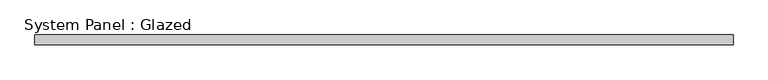
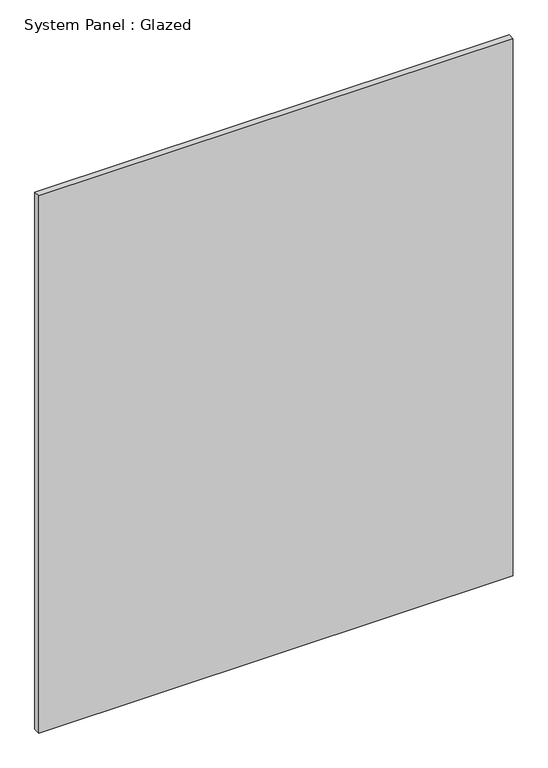
"""IFC4 building model written with IfcOpenShell, lengths in millimetres: plate geometry, System Panel : Glazed."""

from ifc_helpers import new_model, si_unit, origin, origin_with_axes, place, context, project, spatial, polyline, outline, extrude, source, transform, mapped, element, save


def system_panel_glazed_fd736ec2(model_context):
    return source(origin(), model_context, "Body", "SweptSolid", [
        extrude(outline(polyline([(887.9485033, -49.5), (-887.9485033, -49.5), (-887.9485033, -24.5), (887.9485033, -24.5), (887.9485033, -49.5)])), origin_with_axes(), (0.0, 0.0, 1.0), 2125.0),
    ])


if __name__ == "__main__":
    model = new_model("IFC4")
    model_context = context("Model", 3, world=origin())
    ifc_project = project(units=[si_unit("LENGTHUNIT", "METRE", prefix="MILLI")], contexts=[model_context])
    site = spatial("IfcSite", under=ifc_project)
    building = spatial("IfcBuilding", under=site)
    placement = place(None, origin())
    system_panel_glazed_shape = system_panel_glazed_fd736ec2(model_context)
    element("IfcPlate", 1, ObjectType="System Panel : Glazed", at=placement, inside=building, context=model_context, shape_type="MappedRepresentation", body=[
        mapped(system_panel_glazed_shape, transform((0.0, 0.0, 0.0), x_axis=(1.0, 0.0, 0.0), y_axis=(0.0, 1.0, 0.0), z_axis=(0.0, 0.0, 1.0))),
    ])
    save(model, "model.ifc")

# Revit data of these elements
# Type "System Panel : Glazed"
#   Keynote = "H11"
#   Construction Type Id = "GSP4R"
#   Analytic Construction = "1/8 in Pilkington single glazing"
#   Visual Light Transmittance = 0.9
#   Solar Heat Gain Coefficient = 0.86
#   Heat Transfer Coefficient (U) = 6.7069 W/(m²·K)
# Element 1 (IfcPlate, "System Panel : Glazed")
#   Materials on its faces: "Glass"
# Materials
#   "Glass": class "Glass", colour RGB 0 128 192, transparency 0.9, Description = "Soda Lime Glass", Cost = 0
